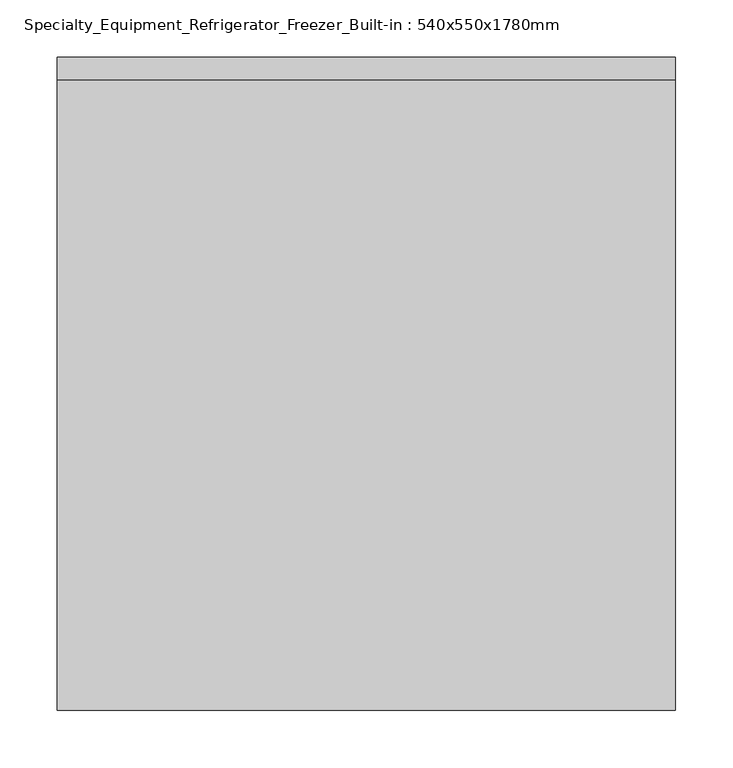
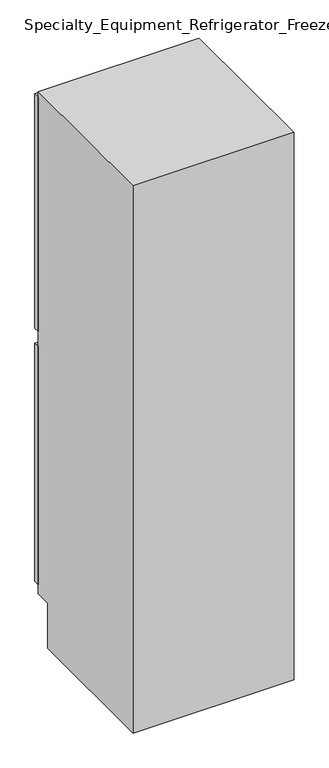
"""IFC4 building model written with IfcOpenShell, lengths in millimetres: proxy geometry, Specialty_Equipment_Refrigerator_Freezer_Built-in : 540x550x1780mm."""

import ifcopenshell
import ifcopenshell.guid

model = None  # the IFC model being written
_history = None  # IfcOwnerHistory: only IFC2X3 demands one
_inside = {}  # id of a spatial element -> (the spatial element, [elements in it])
_under = {}  # id of a project, library or spatial element -> (it, [spatial elements below it])
_declared = {}  # id of a project -> (the project, [libraries it declares])
_typed = {}  # id of a type object -> (the type object, [elements of that type])
_made_of = {}  # id of a material, layer set ... -> (it, [elements and type objects made of it])


def new_model(schema):
    """Start an empty IFC model of exactly this schema.

    Asked for "IFC4X3", IfcOpenShell would pick the latest addendum, in which some entities
    have other attributes; the version numbers below select the first issue.
    IFC2X3 requires an IfcOwnerHistory on every rooted entity: one is made here for all.
    """
    global model, _history
    if schema == "IFC4X3":
        model = ifcopenshell.file(schema_version=(4, 3, 0, 0))
    else:
        model = ifcopenshell.file(schema=schema)
    _inside.clear()
    _under.clear()
    _declared.clear()
    _typed.clear()
    _made_of.clear()
    _history = None
    if model.schema == "IFC2X3":
        org = make("IfcOrganization", Name="unknown")
        user = make(
            "IfcPersonAndOrganization",
            ThePerson=make("IfcPerson", FamilyName="unknown"),
            TheOrganization=org,
        )
        app = make(
            "IfcApplication",
            ApplicationDeveloper=org,
            Version="unknown",
            ApplicationFullName="unknown",
            ApplicationIdentifier="unknown",
        )
        _history = make(
            "IfcOwnerHistory",
            OwningUser=user,
            OwningApplication=app,
            ChangeAction="ADDED",
            CreationDate=0,
        )
    return model


def make(cls, **values):
    """One entity of the class cls with the attributes given. An attribute that is None is left unset."""
    return model.create_entity(
        cls, **{name: value for name, value in values.items() if value is not None}
    )


def rooted(cls, **values):
    """An entity with a GlobalId (a new one), such as an element, a storey or a relation."""
    return make(cls, GlobalId=ifcopenshell.guid.new(), OwnerHistory=_history, **values)


def si_unit(unit_type, name, prefix=None):
    """IfcSIUnit, for example si_unit("LENGTHUNIT", "METRE", prefix="MILLI")."""
    return make("IfcSIUnit", UnitType=unit_type, Prefix=prefix, Name=name)


def assignment(units):
    """IfcUnitAssignment: the units of a project."""
    return None if units is None else make("IfcUnitAssignment", Units=units)


def point(xyz):
    """IfcCartesianPoint."""
    return None if xyz is None else make("IfcCartesianPoint", Coordinates=xyz)


def direction(xyz):
    """IfcDirection."""
    return None if xyz is None else make("IfcDirection", DirectionRatios=xyz)


def frame(location, z_axis=None, x_axis=None):
    """IfcAxis2Placement3D, a coordinate frame: its origin and axes. An axis left out is left unset."""
    return make(
        "IfcAxis2Placement3D",
        Location=point(location),
        Axis=direction(z_axis),
        RefDirection=direction(x_axis),
    )


def origin():
    """The frame at (0, 0, 0) with its axes left unset."""
    return frame((0.0, 0.0, 0.0))


def place(relative_to, where):
    """IfcLocalPlacement: puts the frame where relative to a parent placement (None: the world)."""
    return make(
        "IfcLocalPlacement", PlacementRelTo=relative_to, RelativePlacement=where
    )


def context(
    kind, dimensions, precision=None, world=None, true_north=None, identifier=None
):
    """IfcGeometricRepresentationContext, for example the 3D "Model" context."""
    return make(
        "IfcGeometricRepresentationContext",
        ContextIdentifier=identifier,
        ContextType=kind,
        CoordinateSpaceDimension=dimensions,
        Precision=precision,
        WorldCoordinateSystem=world,
        TrueNorth=true_north,
    )


def project(units=None, contexts=None):
    """IfcProject with its units and contexts."""
    return rooted(
        "IfcProject",
        Name="project",
        RepresentationContexts=contexts,
        UnitsInContext=assignment(units),
    )


def spatial(cls, under=None, at=None, **own):
    """A site, building, storey or space (cls), placed at a placement, below another one or the project."""
    s = rooted(cls, ObjectPlacement=at, **own)
    if under is not None:
        _under.setdefault(under.id(), (under, []))[1].append(s)
    return s


def polyline(points):
    """IfcPolyline through the points."""
    return make("IfcPolyline", Points=[point(p) for p in points])


def outline(outer, holes=None, kind="AREA"):
    """IfcArbitraryClosedProfileDef: a profile drawn as a closed curve; with holes, ...WithVoids."""
    if holes is None:
        return make("IfcArbitraryClosedProfileDef", ProfileType=kind, OuterCurve=outer)
    return make(
        "IfcArbitraryProfileDefWithVoids",
        ProfileType=kind,
        OuterCurve=outer,
        InnerCurves=holes,
    )


def extrude(swept, where, along, depth):
    """IfcExtrudedAreaSolid: the profile swept, set in the frame where, extruded along a direction by depth."""
    return make(
        "IfcExtrudedAreaSolid",
        SweptArea=swept,
        Position=where,
        ExtrudedDirection=direction(along),
        Depth=depth,
    )


def shape(context_of_items, identifier, shape_type, items):
    """IfcShapeRepresentation: the items that make up one representation, for example the "Body"."""
    return make(
        "IfcShapeRepresentation",
        ContextOfItems=context_of_items,
        RepresentationIdentifier=identifier,
        RepresentationType=shape_type,
        Items=items,
    )


def source(mapping_origin, context_of_items, identifier, shape_type, items):
    """IfcRepresentationMap: a shape defined once, which mapped items show again and again."""
    return make(
        "IfcRepresentationMap",
        MappingOrigin=mapping_origin,
        MappedRepresentation=shape(context_of_items, identifier, shape_type, items),
    )


def transform(
    local_origin,
    x_axis=None,
    y_axis=None,
    z_axis=None,
    scale=None,
    scale2=None,
    scale3=None,
    uniform=True,
):
    """IfcCartesianTransformationOperator3D, or its non-uniform kind. x_axis, y_axis, z_axis: its Axis1, 2, 3."""
    if uniform:
        return make(
            "IfcCartesianTransformationOperator3D",
            Axis1=direction(x_axis),
            Axis2=direction(y_axis),
            LocalOrigin=point(local_origin),
            Scale=scale,
            Axis3=direction(z_axis),
        )
    return make(
        "IfcCartesianTransformationOperator3DnonUniform",
        Axis1=direction(x_axis),
        Axis2=direction(y_axis),
        LocalOrigin=point(local_origin),
        Scale=scale,
        Axis3=direction(z_axis),
        Scale2=scale2,
        Scale3=scale3,
    )


def mapped(mapping_source, mapping_target):
    """IfcMappedItem: shows the shape of a source again, moved by a transform."""
    return make(
        "IfcMappedItem", MappingSource=mapping_source, MappingTarget=mapping_target
    )


def made_of(thing, what):
    """Note that an element or type object is made of a material, layer set ...; save() writes the relation."""
    if what is not None:
        _made_of.setdefault(what.id(), (what, []))[1].append(thing)
    return thing


def element(
    cls,
    number,
    at=None,
    inside=None,
    cuts=None,
    type_object=None,
    material=None,
    context=None,
    identifier="Body",
    shape_type=None,
    held_by="IfcProductDefinitionShape",
    body=None,
    shapes=None,
    **own,
):
    """One element of the class cls, such as IfcWall. Its Tag is "e" and its number.

    at: its placement. inside: the storey or other place that contains it. cuts: it is an
    opening in that element (IfcRelVoidsElement). A single representation is given by context,
    identifier, shape_type and body (its items); several are given by shapes. held_by: the class
    of the entity that holds the representations. save() writes the other relations.
    """
    e = rooted(cls, Tag="e%d" % number, ObjectPlacement=at, **own)
    if body is not None:
        shapes = [shape(context, identifier, shape_type, body)]
    if shapes is not None:
        e.Representation = make(held_by, Representations=shapes)
    if inside is not None:
        _inside.setdefault(inside.id(), (inside, []))[1].append(e)
    if cuts is not None:
        rooted(
            "IfcRelVoidsElement", RelatingBuildingElement=cuts, RelatedOpeningElement=e
        )
    if type_object is not None:
        _typed.setdefault(type_object.id(), (type_object, []))[1].append(e)
    return made_of(e, material)


def aggregate(whole, parts):
    """IfcRelAggregates: a whole, such as a stair, and the parts it consists of."""
    return rooted("IfcRelAggregates", RelatingObject=whole, RelatedObjects=parts)


def save(model, path):
    """Write the relations noted so far, then the file.

    IfcRelAggregates (storeys below a building ...), IfcRelContainedInSpatialStructure (elements
    in a storey), IfcRelDefinesByType, IfcRelAssociatesMaterial and IfcRelDeclares: one each for
    every whole, place, type object, material and project.
    """
    for whole, parts in _under.values():
        aggregate(whole, parts)
    for where, things in _inside.values():
        rooted(
            "IfcRelContainedInSpatialStructure",
            RelatedElements=things,
            RelatingStructure=where,
        )
    for kind, things in _typed.values():
        rooted("IfcRelDefinesByType", RelatedObjects=things, RelatingType=kind)
    for what, things in _made_of.values():
        rooted("IfcRelAssociatesMaterial", RelatedObjects=things, RelatingMaterial=what)
    for by, libraries in _declared.values():
        rooted("IfcRelDeclares", RelatingContext=by, RelatedDefinitions=libraries)
    model.write(path)


def specialty_equipment_refrigerator_freezer_built_in_e59dad0f(model_context):
    return source(origin(), model_context, "Body", "SweptSolid", [
        extrude(outline(polyline([(-371.2552993, 786.25), (168.7447007, 786.25), (168.7447007, 766.25), (-371.2552993, 766.25), (-371.2552993, 786.25)])), frame((0.0, 0.0, 1090.0), z_axis=(0.0, 0.0, 1.0), x_axis=(1.0, 0.0, 0.0)), (0.0, 0.0, 1.0), 830.0),
        extrude(outline(polyline([(-371.2552993, 786.25), (168.7447007, 786.25), (168.7447007, 766.25), (-371.2552993, 766.25), (-371.2552993, 786.25)])), frame((0.0, 0.0, 192.0), z_axis=(0.0, 0.0, 1.0), x_axis=(1.0, 0.0, 0.0)), (0.0, 0.0, 1.0), 845.0),
        extrude(outline(polyline([(711.0710563, 0.0), (216.25, 0.0), (216.25, 1940.0), (766.25, 1940.0), (766.25, 160.0), (711.0710563, 160.0), (711.0710563, 0.0)])), frame((-371.2552993, 0.0, 0.0), z_axis=(1.0, 0.0, 0.0), x_axis=(0.0, 1.0, 0.0)), (0.0, 0.0, 1.0), 540.0),
    ])


if __name__ == "__main__":
    model = new_model("IFC4")
    model_context = context("Model", 3, world=origin())
    ifc_project = project(units=[si_unit("LENGTHUNIT", "METRE", prefix="MILLI")], contexts=[model_context])
    site = spatial("IfcSite", under=ifc_project)
    building = spatial("IfcBuilding", under=site)
    placement = place(None, origin())
    specialty_equipment_refrigerator_freezer_built_in_shape = specialty_equipment_refrigerator_freezer_built_in_e59dad0f(model_context)
    element("IfcBuildingElementProxy", 1, Name="Specialty_Equipment_Refrigerator_Freezer_Built-in : 540x550x1780mm", ObjectType="Specialty_Equipment_Refrigerator_Freezer_Built-in : 540x550x1780mm", at=placement, inside=building, context=model_context, shape_type="MappedRepresentation", body=[
        mapped(specialty_equipment_refrigerator_freezer_built_in_shape, transform((0.0, 0.0, 0.0), x_axis=(1.0, 0.0, 0.0), y_axis=(0.0, 1.0, 0.0), z_axis=(0.0, 0.0, 1.0))),
    ])
    save(model, "model.ifc")

# Revit data of these elements
# Type "Specialty_Equipment_Refrigerator_Freezer_Built-in : 540x550x1780mm"
#   Label = "REF."
#   Keynote = "N"
#   Depth = 550 mm
#   Height = 1780 mm
#   Plinth Height = 160 mm
#   Width = 540 mm
#   Material = Metal - Paint Finish - Ivory, Glossy
#   Default Elevation = 0
# Element 1 (IfcBuildingElementProxy, "Specialty_Equipment_Refrigerator_Freezer_Built-in : 540x550x1780mm")
#   Materials on its faces: "Metal - Paint Finish - Ivory, Glossy"
# Materials
#   "Metal - Paint Finish - Ivory, Glossy": class "Paint", colour RGB 247 247 239, transparency 0
